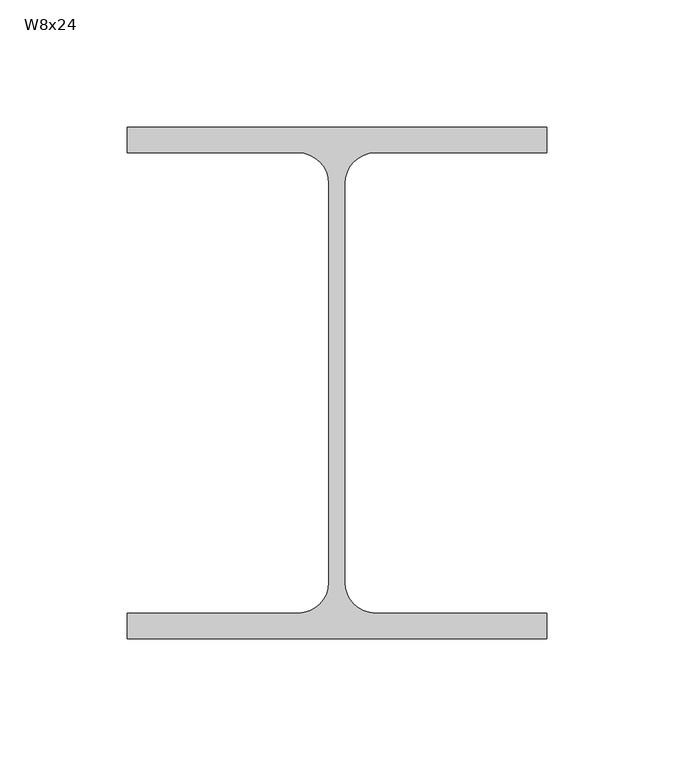
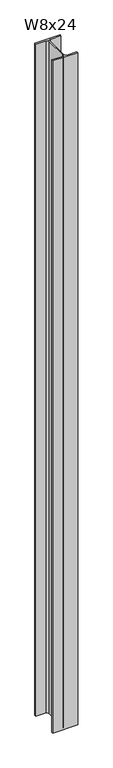
"""IFC4 building model written with IfcOpenShell, lengths in millimetres: column geometry, RME WF - Column : W8x24."""

from ifc_helpers import new_model, si_unit, point, frame_2d, origin, origin_with_axes, place, context, project, spatial, polyline, circle_curve, trimmed, segment, composite_curve, outline, extrude, source, transform, mapped, element, save


def w8x24_af725de8(model_context):
    return source(origin(), model_context, "Body", "SweptSolid", [
        extrude(outline(composite_curve([segment(polyline([(82.55, 100.711), (82.55, 90.551), (15.1765, 90.551)]), True, "CONTINUOUS"), segment(trimmed(circle_curve(frame_2d((15.1765, 78.486)), 12.065), [point((15.1765, 90.551))], [point((3.1115, 78.486))], True, "CARTESIAN"), True, "CONTINUOUS"), segment(polyline([(3.1115, 78.486), (3.1115, -78.486)]), True, "CONTINUOUS"), segment(trimmed(circle_curve(frame_2d((15.1765, -78.486)), 12.065), [point((3.1115, -78.486))], [point((15.1765, -90.551))], True, "CARTESIAN"), True, "CONTINUOUS"), segment(polyline([(15.1765, -90.551), (82.55, -90.551), (82.55, -100.711), (-82.55, -100.711), (-82.55, -90.551), (-15.1765, -90.551)]), True, "CONTINUOUS"), segment(trimmed(circle_curve(frame_2d((-15.1765, -78.486)), 12.065), [point((-15.1765, -90.551))], [point((-3.1115, -78.486))], True, "CARTESIAN"), True, "CONTINUOUS"), segment(polyline([(-3.1115, -78.486), (-3.1115, 78.486)]), True, "CONTINUOUS"), segment(trimmed(circle_curve(frame_2d((-15.1765, 78.486)), 12.065), [point((-3.1115, 78.486))], [point((-15.1765, 90.551))], True, "CARTESIAN"), True, "CONTINUOUS"), segment(polyline([(-15.1765, 90.551), (-82.55, 90.551), (-82.55, 100.711), (82.55, 100.711)]), True, "CONTINUOUS")], self_intersect=False)), origin_with_axes(), (0.0, 0.0, 1.0), 4660.9),
    ])


if __name__ == "__main__":
    model = new_model("IFC4")
    model_context = context("Model", 3, world=origin())
    ifc_project = project(units=[si_unit("LENGTHUNIT", "METRE", prefix="MILLI")], contexts=[model_context])
    site = spatial("IfcSite", under=ifc_project)
    building = spatial("IfcBuilding", under=site)
    placement = place(None, origin())
    w8x24_shape = w8x24_af725de8(model_context)
    element("IfcColumn", 1, ObjectType="RME WF - Column : W8x24", at=placement, inside=building, context=model_context, shape_type="MappedRepresentation", body=[
        mapped(w8x24_shape, transform((0.0, 0.0, 0.0), x_axis=(1.0, 0.0, 0.0), y_axis=(0.0, 1.0, 0.0), z_axis=(0.0, 0.0, 1.0))),
    ])
    save(model, "model.ifc")

# Revit data of these elements
# Type "RME WF - Column : W8x24"
#   Type Mark = "C1"
#   REINF TYPE [instance default] = ""
#   Nominal Size = "W16"
#   COL REMARKS [instance default] = ""
#   BP [instance default] = ""
#   Assembly Code = "B10"
#   W = 24
#   bf = 0' - 6 1/2"
#   d = 0' - 7.93"
#   k = 0' - 0 7/8"
#   kr = 0' - 0.475"
#   tf = 0' - 0.4"
#   tw = 0' - 0.245"
#   A = 0.0491667 SF
#   Structural Material [instance default] = Metal - Steel - ASTM A992
# Element 1 (IfcColumn, "RME WF - Column : W8x24")
#   Materials on its faces: "Metal - Steel - ASTM A992"
# Materials
#   "Metal - Steel - ASTM A992": class "Metal", colour RGB 255 128 0, transparency 0
